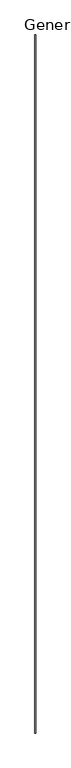
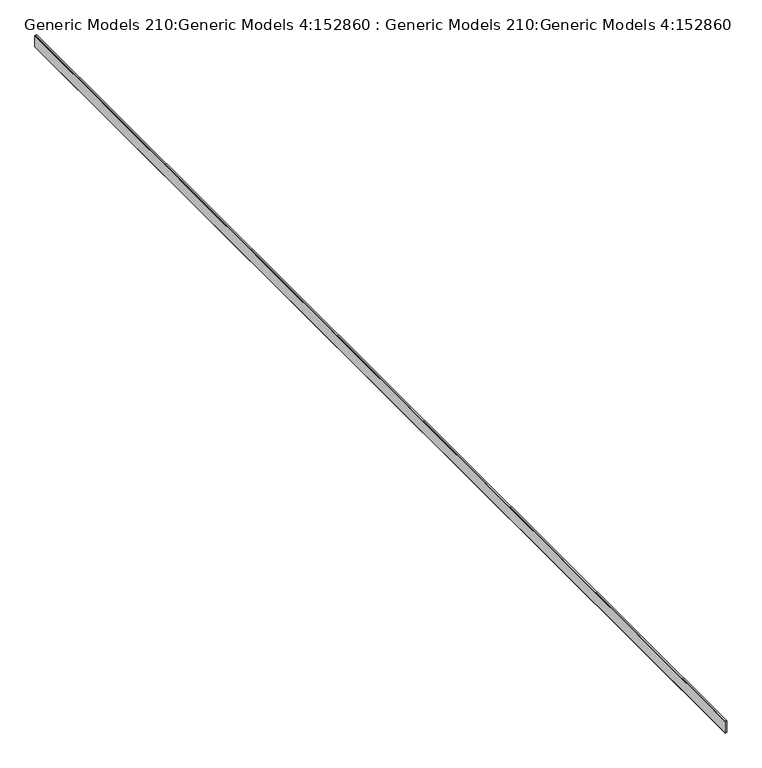
"""IFC4 building model written with IfcOpenShell, lengths in millimetres: proxy geometry, Generic Models 210:Generic Models 4:152860 : Generic Models 210:Generic Models 4:152860."""

from ifc_helpers import new_model, si_unit, frame, origin, place, context, project, spatial, polyline, outline, extrude, source, transform, mapped, element, save


def generic_models_210_generic_models_4_152860_generic_models_676fcff4(model_context):
    return source(origin(), model_context, "Body", "SweptSolid", [
        extrude(outline(polyline([(2896.6618287, -6688.0343913), (2896.6618287, -6670.9844166), (3024.505, -6670.9844166), (3024.505, -6688.0343913), (3021.0252, -6688.0343913), (3021.0252, -6689.3043913), (2900.1416287, -6689.3043913), (2900.1416287, -6688.4455504), (2919.1862074, -6688.4455504), (2919.1862074, -6687.1755504), (2898.8716287, -6687.1755504), (2898.8716287, -6688.0343913), (2896.6618287, -6688.0343913)])), frame((0.0, -273.9974793, 0.0), z_axis=(0.0, 1.0, 0.0), x_axis=(0.0, 0.0, 1.0)), (0.0, 0.0, 1.0), 12242.8),
    ])


if __name__ == "__main__":
    model = new_model("IFC4")
    model_context = context("Model", 3, world=origin())
    ifc_project = project(units=[si_unit("LENGTHUNIT", "METRE", prefix="MILLI")], contexts=[model_context])
    site = spatial("IfcSite", under=ifc_project)
    building = spatial("IfcBuilding", under=site)
    placement = place(None, origin())
    generic_models_210_generic_models_4_152860_generic_models_shape = generic_models_210_generic_models_4_152860_generic_models_676fcff4(model_context)
    element("IfcBuildingElementProxy", 1, Name="Generic Models 210:Generic Models 4:152860 : Generic Models 210:Generic Models 4:152860", ObjectType="Generic Models 210:Generic Models 4:152860 : Generic Models 210:Generic Models 4:152860", at=placement, inside=building, context=model_context, shape_type="MappedRepresentation", body=[
        mapped(generic_models_210_generic_models_4_152860_generic_models_shape, transform((0.0, 0.0, 0.0), x_axis=(1.0, 0.0, 0.0), y_axis=(0.0, 1.0, 0.0), z_axis=(0.0, 0.0, 1.0))),
    ])
    save(model, "model.ifc")

# Revit data of these elements
# Type "Generic Models 210:Generic Models 4:152860 : Generic Models 210:Generic Models 4:152860"
#   NameOverride = "Generic Models 210:Generic Models 4:152860"
#   ObjectTypeOverride = "Generic Models 210:Generic Models 4"
#   Reference = "Generic Models 4"
#   Category = "Generic Models"
#   Tag = "152860"
# Element 1 (IfcBuildingElementProxy, "Generic Models 210:Generic Models 4:152860 : Generic Models 210:Generic Models 4:152860")
#   Materials on its faces: "_7/8\" SMOOTH TROWEL EXTERIOR STUCCO (COLOR PER OWNER) 770"
# Materials
#   "_7/8\" SMOOTH TROWEL EXTERIOR STUCCO (COLOR PER OWNER) 770": class "Unassigned", colour RGB 233 233 233, transparency 0
